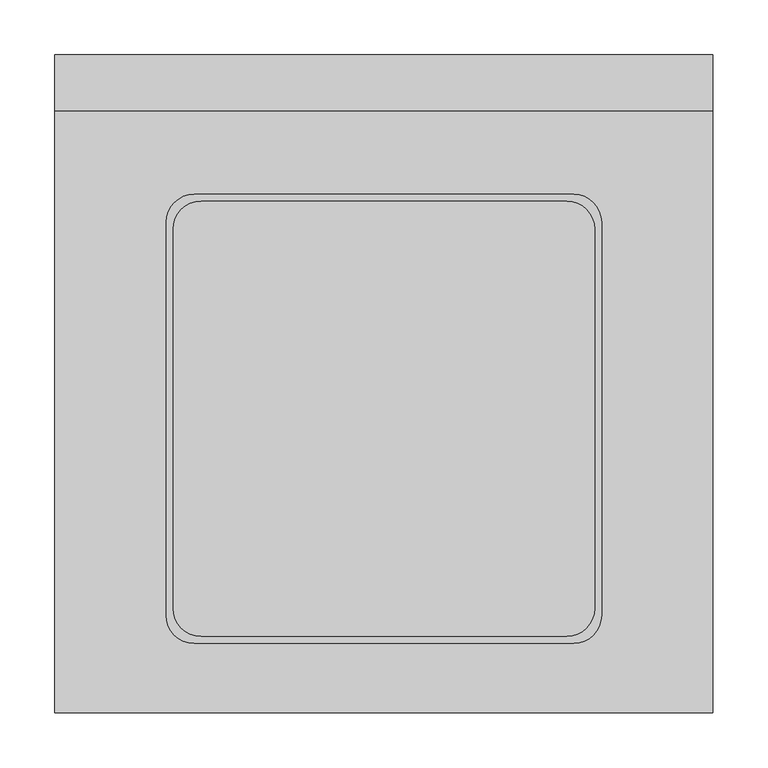
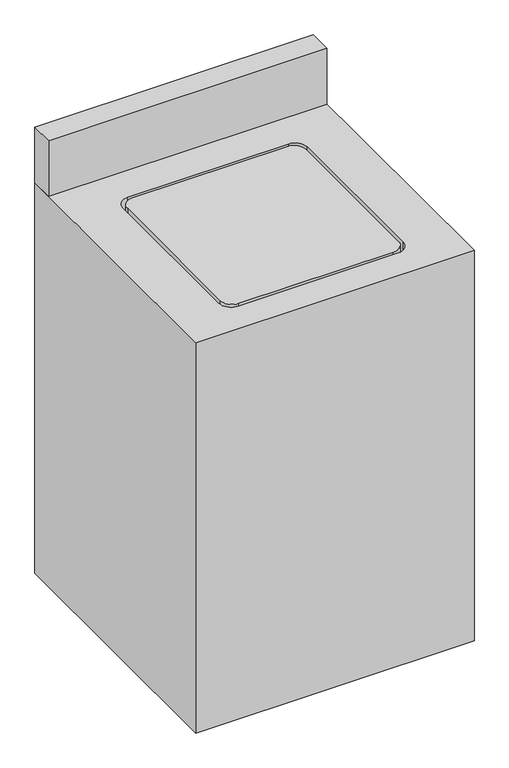
"""IFC4 building model written with IfcOpenShell, lengths in millimetres: proxy geometry, .LAVA-ROUPAS : Lava-roupas."""

from ifc_helpers import new_model, si_unit, point, frame, frame_2d, origin, place, context, project, spatial, polyline, circle_curve, trimmed, segment, composite_curve, outline, extrude, source, transform, mapped, element, save
from ifc_brep_helpers import plane_surface, revolved_surface, advanced_brep


def specialty_equipment_0c7a4015(model_context):
    return source(origin(), model_context, "Body", "SolidModel", [
        extrude(outline(composite_curve([segment(trimmed(circle_curve(frame_2d((210.8674685, 437.8995648)), 25.4), [point((185.4674685, 437.8995648))], [point((210.8674685, 463.2995648))], False, "CARTESIAN"), True, "CONTINUOUS"), segment(polyline([(210.8674685, 463.2995648), (544.1674685, 463.2995648)]), True, "CONTINUOUS"), segment(trimmed(circle_curve(frame_2d((544.1674685, 437.8995648)), 25.4), [point((544.1674685, 463.2995648))], [point((569.5674685, 437.8995648))], False, "CARTESIAN"), True, "CONTINUOUS"), segment(polyline([(569.5674685, 437.8995648), (569.5674685, 91.8995648)]), True, "CONTINUOUS"), segment(trimmed(circle_curve(frame_2d((544.1674685, 91.8995648)), 25.4), [point((569.5674685, 91.8995648))], [point((544.1674685, 66.4995648))], False, "CARTESIAN"), True, "CONTINUOUS"), segment(polyline([(544.1674685, 66.4995648), (210.8674685, 66.4995648)]), True, "CONTINUOUS"), segment(trimmed(circle_curve(frame_2d((210.8674685, 91.8995648)), 25.4), [point((210.8674685, 66.4995648))], [point((185.4674685, 91.8995648))], False, "CARTESIAN"), True, "CONTINUOUS"), segment(polyline([(185.4674685, 91.8995648), (185.4674685, 437.8995648)]), True, "CONTINUOUS")], self_intersect=False)), frame((0.0, 0.0, 864.6), z_axis=(0.0, 0.0, 1.0), x_axis=(1.0, 0.0, 0.0)), (0.0, 0.0, 1.0), 25.4),
        extrude(outline(polyline([(77.5174685, 545.8495648), (77.5174685, 596.6495648), (677.5174685, 596.6495648), (677.5174685, 545.8495648), (77.5174685, 545.8495648)])), frame((0.0, 0.0, 890.0), z_axis=(0.0, 0.0, 1.0), x_axis=(1.0, 0.0, 0.0)), (0.0, 0.0, 1.0), 127.0),
        advanced_brep(
        [(77.5174685, 596.6495648, 890.0), (77.5174685, -3.3504352, 890.0), (677.5174685, -3.3504352, 890.0), (677.5174685, 596.6495648, 890.0), (204.5174685, 469.4681955, 890.0), (550.5174685, 469.4681955, 890.0), (575.9174685, 444.0681955, 890.0), (575.9174685, 85.5495648, 890.0), (550.5174685, 60.1495648, 890.0), (204.5174685, 60.1495648, 890.0), (179.1174685, 85.5495648, 890.0), (179.1174685, 444.0681955, 890.0), (77.5174685, 596.6495648, 0.0), (677.5174685, 596.6495648, 0.0), (677.5174685, -3.3504352, 0.0), (77.5174685, -3.3504352, 0.0), (550.5174685, 469.4681955, 839.2), (204.5174685, 469.4681955, 839.2), (179.1174685, 444.0681955, 839.2), (179.1174685, 85.5495648, 839.2), (204.5174685, 60.1495648, 839.2), (550.5174685, 60.1495648, 839.2), (575.9174685, 85.5495648, 839.2), (575.9174685, 444.0681955, 839.2)],
        [
            (0, 1),
            (1, 2),
            (2, 3),
            (3, 0),
            (4, 5),
            (5, 6, circle_curve(frame((550.5174685, 444.0681955, 890.0), z_axis=(0.0, 0.0, -1.0), x_axis=(0.0, -1.0, 0.0)), 25.4)),
            (6, 7),
            (7, 8, circle_curve(frame((550.5174685, 85.5495648, 890.0), z_axis=(0.0, 0.0, -1.0), x_axis=(0.0, -1.0, 0.0)), 25.4)),
            (8, 9),
            (9, 10, circle_curve(frame((204.5174685, 85.5495648, 890.0), z_axis=(0.0, 0.0, -1.0), x_axis=(0.0, -1.0, 0.0)), 25.4)),
            (10, 11),
            (11, 4, circle_curve(frame((204.5174685, 444.0681955, 890.0), z_axis=(0.0, 0.0, -1.0), x_axis=(0.0, -1.0, 0.0)), 25.4)),
            (12, 13),
            (13, 14),
            (14, 15),
            (15, 12),
            (0, 12),
            (15, 1),
            (14, 2),
            (13, 3),
            (16, 17),
            (17, 18, circle_curve(frame((204.5174685, 444.0681955, 839.2), z_axis=(0.0, 0.0, 1.0), x_axis=(0.0, -1.0, 0.0)), 25.4)),
            (18, 19),
            (19, 20, circle_curve(frame((204.5174685, 85.5495648, 839.2), z_axis=(0.0, 0.0, 1.0), x_axis=(0.0, -1.0, 0.0)), 25.4)),
            (20, 21),
            (21, 22, circle_curve(frame((550.5174685, 85.5495648, 839.2), z_axis=(0.0, 0.0, 1.0), x_axis=(0.0, -1.0, 0.0)), 25.4)),
            (22, 23),
            (23, 16, circle_curve(frame((550.5174685, 444.0681955, 839.2), z_axis=(0.0, 0.0, 1.0), x_axis=(0.0, -1.0, 0.0)), 25.4)),
            (16, 5),
            (4, 17),
            (11, 18),
            (10, 19),
            (9, 20),
            (8, 21),
            (7, 22),
            (6, 23),
        ],
        [
            plane_surface(frame((77.5174685, -3.3504352, 890.0), z_axis=(0.0, 0.0, 1.0), x_axis=(0.0, -1.0, 0.0))),
            plane_surface(frame((77.5174685, -3.3504352, 0.0), z_axis=(0.0, 0.0, -1.0), x_axis=(0.0, 1.0, 0.0))),
            plane_surface(frame((77.5174685, 596.6495648, 890.0), z_axis=(-1.0, 0.0, 0.0), x_axis=(0.0, 0.0, -1.0))),
            plane_surface(frame((77.5174685, -3.3504352, 890.0), z_axis=(0.0, -1.0, 0.0), x_axis=(0.0, 0.0, -1.0))),
            plane_surface(frame((677.5174685, -3.3504352, 890.0), z_axis=(1.0, 0.0, 0.0), x_axis=(0.0, 0.0, -1.0))),
            plane_surface(frame((677.5174685, 596.6495648, 890.0), z_axis=(0.0, 1.0, 0.0), x_axis=(0.0, 0.0, -1.0))),
            plane_surface(frame((204.5174685, 469.4681955, 839.2), z_axis=(0.0, 0.0, 1.0), x_axis=(1.0, 0.0, 0.0))),
            plane_surface(frame((550.5174685, 469.4681955, 890.0), z_axis=(0.0, -1.0, 0.0), x_axis=(0.0, 0.0, -1.0))),
            revolved_surface(polyline([(204.5174685, 418.6681955, 890.0), (204.5174685, 418.6681955, 839.2)]), (204.5174685, 444.0681955, 839.2), (0.0, 0.0, 1.0)),
            plane_surface(frame((179.1174685, 444.0681955, 890.0), z_axis=(1.0, 0.0, 0.0), x_axis=(0.0, 0.0, -1.0))),
            revolved_surface(polyline([(204.5174685, 60.1495648, 890.0), (204.5174685, 60.1495648, 839.2)]), (204.5174685, 85.5495648, 839.2), (0.0, 0.0, 1.0)),
            plane_surface(frame((204.5174685, 60.1495648, 890.0), z_axis=(0.0, 1.0, 0.0), x_axis=(0.0, 0.0, -1.0))),
            revolved_surface(polyline([(550.5174685, 60.1495648, 890.0), (550.5174685, 60.1495648, 839.2)]), (550.5174685, 85.5495648, 839.2), (0.0, 0.0, 1.0)),
            plane_surface(frame((575.9174685, 85.5495648, 890.0), z_axis=(-1.0, 0.0, 0.0), x_axis=(0.0, 0.0, -1.0))),
            revolved_surface(polyline([(550.5174685, 418.6681955, 890.0), (550.5174685, 418.6681955, 839.2)]), (550.5174685, 444.0681955, 839.2), (0.0, 0.0, 1.0)),
        ],
        [
            (0, [[1, 2, 3, 4], [5, 6, 7, 8, 9, 10, 11, 12]]),
            (1, [[13, 14, 15, 16]]),
            (2, [[-1, 17, -16, 18]]),
            (3, [[-2, -18, -15, 19]]),
            (4, [[-3, -19, -14, 20]]),
            (5, [[-4, -20, -13, -17]]),
            (6, [[21, 22, 23, 24, 25, 26, 27, 28]]),
            (7, [[-21, 29, -5, 30]]),
            (8, [[-22, -30, -12, 31]]),
            (9, [[-23, -31, -11, 32]]),
            (10, [[-24, -32, -10, 33]]),
            (11, [[-25, -33, -9, 34]]),
            (12, [[-26, -34, -8, 35]]),
            (13, [[-27, -35, -7, 36]]),
            (14, [[-28, -36, -6, -29]]),
        ],
    ),
    ])


if __name__ == "__main__":
    model = new_model("IFC4")
    model_context = context("Model", 3, world=origin())
    ifc_project = project(units=[si_unit("LENGTHUNIT", "METRE", prefix="MILLI")], contexts=[model_context])
    site = spatial("IfcSite", under=ifc_project)
    building = spatial("IfcBuilding", under=site)
    placement = place(None, origin())
    specialty_equipment_shape = specialty_equipment_0c7a4015(model_context)
    element("IfcBuildingElementProxy", 1, Name=".LAVA-ROUPAS : Lava-roupas", ObjectType=".LAVA-ROUPAS : Lava-roupas", at=placement, inside=building, context=model_context, shape_type="MappedRepresentation", body=[
        mapped(specialty_equipment_shape, transform((0.0, 0.0, 0.0), x_axis=(1.0, 0.0, 0.0), y_axis=(0.0, 1.0, 0.0), z_axis=(0.0, 0.0, 1.0))),
    ])
    save(model, "model.ifc")

# Revit data of these elements
# Type ".LAVA-ROUPAS : Lava-roupas"
#   Marca = "Brastemp"
#   Profundidade = 0.60 m
#   Altura = 0.89 m
#   Largura = 0.60 m
#   Acabamento = Pintura - marfim
# Element 1 (IfcBuildingElementProxy, ".LAVA-ROUPAS : Lava-roupas")
#   Materials on its faces: "Pintura - marfim"
# Materials
#   "Pintura - marfim": class "Peinture", colour RGB 247 247 239, transparency 0, Cost = 0
